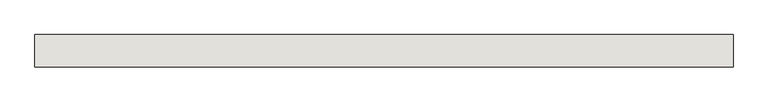
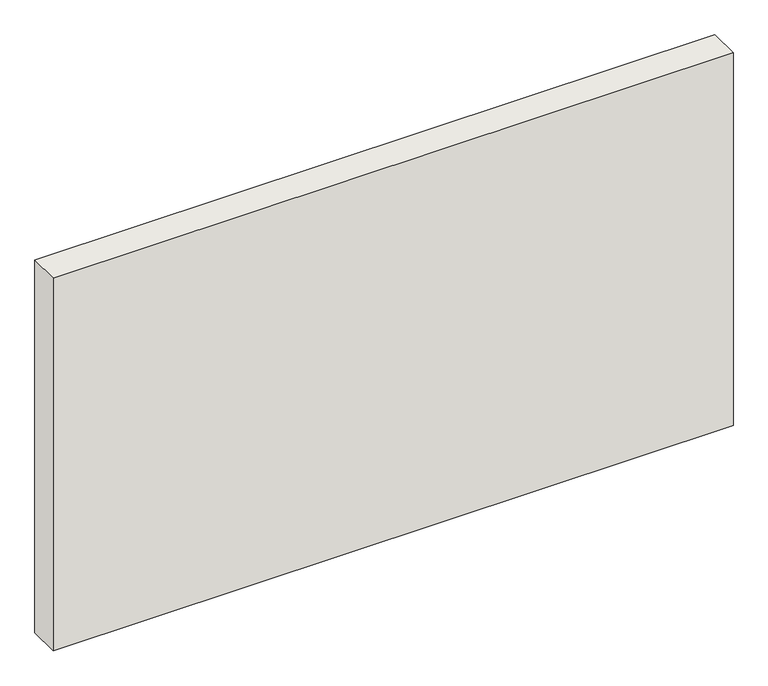
"""IFC4 building model written with IfcOpenShell, lengths in millimetres: wall geometry, Holzwand."""

from ifc_helpers import new_model, si_unit, origin, origin_with_axes, place, context, project, spatial, polyline, outline, extrude, source, transform, mapped, element, save


def wall_b401368d(model_context):
    return source(origin(), model_context, "Body", "SweptSolid", [
        extrude(outline(polyline([(0.0, 200.0), (4327.8619019, 200.0), (4327.8619019, 0.0), (0.0, 0.0), (0.0, 200.0)])), origin_with_axes(), (0.0, 0.0, 1.0), 2510.0),
    ])


if __name__ == "__main__":
    model = new_model("IFC4")
    model_context = context("Model", 3, world=origin())
    ifc_project = project(units=[si_unit("LENGTHUNIT", "METRE", prefix="MILLI")], contexts=[model_context])
    site = spatial("IfcSite", under=ifc_project)
    building = spatial("IfcBuilding", under=site)
    placement = place(None, origin())
    wall_shape = wall_b401368d(model_context)
    element("IfcWall", 1, ObjectType="Holzwand", at=placement, inside=building, context=model_context, shape_type="MappedRepresentation", body=[
        mapped(wall_shape, transform((0.0, 0.0, 0.0), x_axis=(1.0, 0.0, 0.0), y_axis=(0.0, 1.0, 0.0), z_axis=(0.0, 0.0, 1.0))),
    ])
    save(model, "model.ifc")

# Revit data of these elements
# Element 1 (IfcWall, "Holzwand")
#   Materials on its faces: "holzschalung"
# Materials
#   "holzschalung": class "Unassigned", colour RGB 128 128 128, transparency 0
